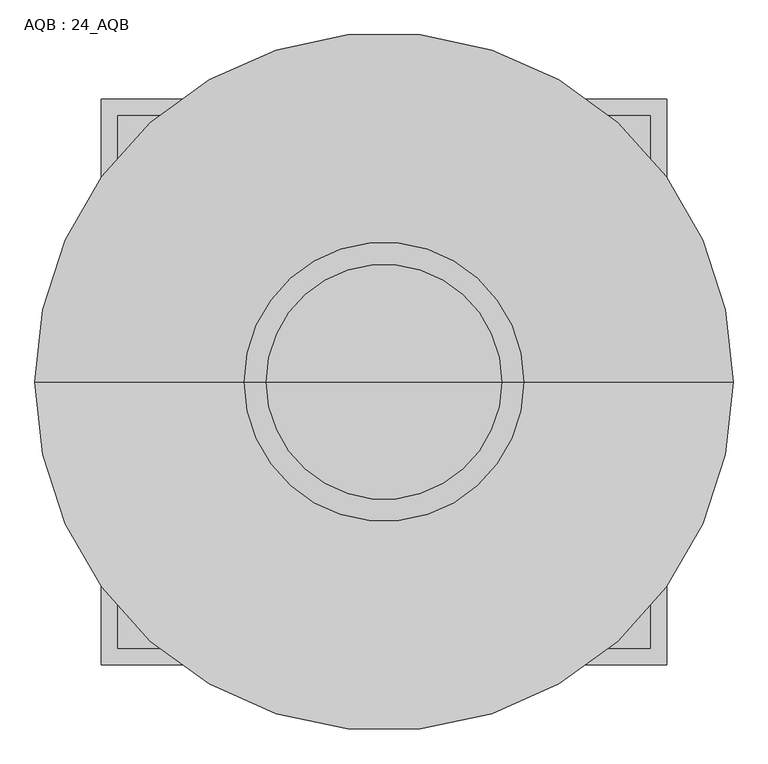
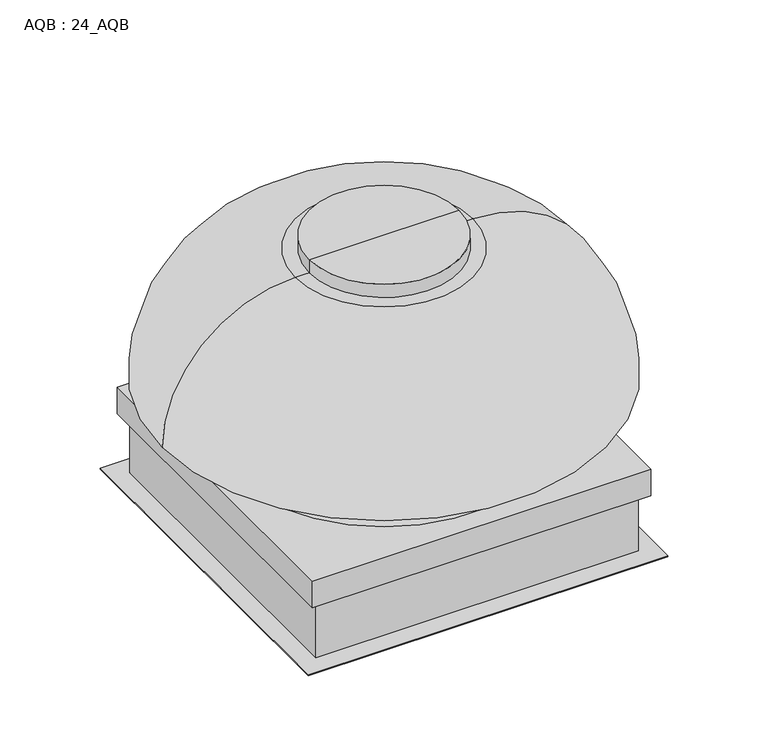
"""IFC4 building model written with IfcOpenShell, lengths in millimetres: proxy geometry, AQB : 24_AQB."""

from ifc_helpers import new_model, si_unit, point, frame, origin, place, context, project, spatial, polyline, circle_curve, ellipse_curve, trimmed, outline, extrude, faceted_brep, source, transform, mapped, element, save
from ifc_brep_helpers import plane_surface, cylinder_surface, revolved_surface, advanced_brep


def aqb_24_aqb_14a4d41b(model_context):
    return source(origin(), model_context, "Body", "SolidModel", [
        extrude(outline(polyline([(499.247472, -488.95), (-478.652528, -488.95), (-478.652528, 488.95), (499.247472, 488.95), (499.247472, -488.95)]), holes=[polyline([(-427.852528, 438.15), (-427.852528, -438.15), (448.447472, -438.15), (448.447472, 438.15), (-427.852528, 438.15)])]), frame((0.0, 0.0, -168.275), z_axis=(0.0, 0.0, 1.0), x_axis=(1.0, 0.0, 0.0)), (0.0, 0.0, 1.0), 3.175),
        extrude(outline(polyline([(-427.852528, 438.15), (448.447472, 438.15), (448.447472, -438.15), (-427.852528, -438.15), (-427.852528, 438.15)]), holes=[polyline([(410.347472, -400.05), (410.347472, 400.05), (-389.752528, 400.05), (-389.752528, -400.05), (410.347472, -400.05)])]), frame((0.0, 0.0, -168.275), z_axis=(0.0, 0.0, 1.0), x_axis=(1.0, 0.0, 0.0)), (0.0, 0.0, 1.0), 241.3),
        advanced_brep(
        [(10.297472, 0.0, 593.725), (-192.902528, 0.0, 593.725), (213.497472, 0.0, 593.725), (213.497472, 0.0, 631.825), (-192.902528, 0.0, 631.825), (10.297472, 0.0, 631.825)],
        [
            (0, 1),
            (1, 2, circle_curve(frame((10.297472, 0.0, 593.725), z_axis=(0.0, 0.0, -1.0), x_axis=(-1.0, 0.0, 0.0)), 203.2)),
            (2, 0),
            (2, 1, circle_curve(frame((10.297472, 0.0, 593.725), z_axis=(0.0, 0.0, -1.0), x_axis=(-1.0, 0.0, 0.0)), 203.2)),
            (3, 4, circle_curve(frame((10.297472, 0.0, 631.825), z_axis=(0.0, 0.0, 1.0), x_axis=(-1.0, 0.0, 0.0)), 203.2)),
            (4, 5),
            (5, 3),
            (4, 3, circle_curve(frame((10.297472, 0.0, 631.825), z_axis=(0.0, 0.0, 1.0), x_axis=(-1.0, 0.0, 0.0)), 203.2)),
            (1, 4),
            (3, 2),
        ],
        [
            plane_surface(frame((10.297472, 0.0, 593.725), z_axis=(0.0, 0.0, -1.0), x_axis=(-1.0, 0.0, 0.0))),
            plane_surface(frame((10.297472, 0.0, 631.825), z_axis=(0.0, 0.0, 1.0), x_axis=(-1.0, 0.0, 0.0))),
            cylinder_surface(frame((10.297472, 0.0, 593.725), z_axis=(0.0, 0.0, -1.0), x_axis=(-1.0, 0.0, 0.0)), 203.2),
        ],
        [
            (0, [[1, 2, 3]]),
            (0, [[-3, 4, -1]]),
            (1, [[5, 6, 7]]),
            (1, [[8, -7, -6]]),
            (2, [[-2, 9, -5, 10]]),
            (2, [[-4, -10, -8, -9]]),
        ],
    ),
        advanced_brep(
        [(10.297472, 0.0, 231.775), (-592.952528, 0.0, 231.775), (613.547472, 0.0, 231.775), (251.597472, 0.0, 593.725), (-231.002528, 0.0, 593.725), (10.297472, 0.0, 593.725)],
        [
            (0, 1),
            (1, 2, circle_curve(frame((10.297472, 0.0, 231.775), z_axis=(0.0, 0.0, -1.0), x_axis=(-1.0, 0.0, 0.0)), 603.25)),
            (2, 0),
            (2, 1, circle_curve(frame((10.297472, 0.0, 231.775), z_axis=(0.0, 0.0, -1.0), x_axis=(-1.0, 0.0, 0.0)), 603.25)),
            (3, 4, circle_curve(frame((10.297472, 0.0, 593.725), z_axis=(0.0, 0.0, 1.0), x_axis=(-1.0, 0.0, 0.0)), 241.3)),
            (4, 5),
            (5, 3),
            (4, 3, circle_curve(frame((10.297472, 0.0, 593.725), z_axis=(0.0, 0.0, 1.0), x_axis=(-1.0, 0.0, 0.0)), 241.3)),
            (1, 4, circle_curve(frame((-231.002528, 0.0, 231.775), z_axis=(0.0, 1.0, 0.0), x_axis=(1.0, 0.0, 0.0)), 361.95)),
            (3, 2, circle_curve(frame((251.597472, 0.0, 231.775), z_axis=(0.0, 1.0, 0.0), x_axis=(-1.0, 0.0, 0.0)), 361.95)),
        ],
        [
            plane_surface(frame((10.297472, 0.0, 231.775), z_axis=(0.0, 0.0, -1.0), x_axis=(-1.0, 0.0, 0.0))),
            plane_surface(frame((10.297472, 0.0, 593.725), z_axis=(0.0, 0.0, 1.0), x_axis=(-1.0, 0.0, 0.0))),
            revolved_surface(trimmed(ellipse_curve(frame((-231.002528, 0.0, 231.775), z_axis=(0.0, -1.0, 0.0), x_axis=(1.0, 0.0, 0.0)), 361.95, 361.95), [point((-231.002528, 0.0, 593.725))], [point((-592.952528, 0.0, 231.775))], True, "CARTESIAN"), (10.297472, 0.0, 593.725), (0.0, 0.0, -1.0)),
        ],
        [
            (0, [[1, 2, 3]]),
            (0, [[-3, 4, -1]]),
            (1, [[5, 6, 7]]),
            (1, [[8, -7, -6]]),
            (2, [[-2, 9, -5, 10]]),
            (2, [[-4, -10, -8, -9]]),
        ],
    ),
        advanced_brep(
        [(416.697472, 0.0, 231.775), (-396.102528, 0.0, 231.775), (10.297472, 0.0, 231.775), (416.697472, 0.0, 76.2), (-396.102528, 0.0, 76.2), (10.297472, 0.0, 76.2)],
        [
            (0, 1, circle_curve(frame((10.297472, 0.0, 231.775), z_axis=(0.0, 0.0, 1.0), x_axis=(-1.0, 0.0, 0.0)), 406.4)),
            (1, 2),
            (2, 0),
            (1, 0, circle_curve(frame((10.297472, 0.0, 231.775), z_axis=(0.0, 0.0, 1.0), x_axis=(-1.0, 0.0, 0.0)), 406.4)),
            (3, 4, circle_curve(frame((10.297472, 0.0, 76.2), z_axis=(0.0, 0.0, 1.0), x_axis=(-1.0, 0.0, 0.0)), 406.4)),
            (4, 1, circle_curve(frame((-396.102528, 0.0, 153.9875), z_axis=(0.0, -1.0, 0.0), x_axis=(1.0, 0.0, 0.0)), 77.7875)),
            (0, 3, circle_curve(frame((416.697472, 0.0, 153.9875), z_axis=(0.0, -1.0, 0.0), x_axis=(-1.0, 0.0, 0.0)), 77.7875)),
            (4, 3, circle_curve(frame((10.297472, 0.0, 76.2), z_axis=(0.0, 0.0, 1.0), x_axis=(-1.0, 0.0, 0.0)), 406.4)),
            (5, 4),
            (3, 5),
        ],
        [
            plane_surface(frame((10.297472, 0.0, 231.775), z_axis=(0.0, 0.0, 1.0), x_axis=(-1.0, 0.0, 0.0))),
            revolved_surface(trimmed(ellipse_curve(frame((-396.102528, 0.0, 153.9875), z_axis=(0.0, 1.0, 0.0), x_axis=(1.0, 0.0, 0.0)), 77.7875, 77.7875), [point((-396.102528, 0.0, 231.775))], [point((-396.102528, 0.0, 76.2))], True, "CARTESIAN"), (10.297472, 0.0, 76.2), (0.0, 0.0, -1.0)),
            plane_surface(frame((10.297472, 0.0, 76.2), z_axis=(0.0, 0.0, -1.0), x_axis=(-1.0, 0.0, 0.0))),
        ],
        [
            (0, [[1, 2, 3]]),
            (0, [[4, -3, -2]]),
            (1, [[5, 6, -1, 7]]),
            (1, [[8, -7, -4, -6]]),
            (2, [[9, -5, 10]]),
            (2, [[-10, -8, -9]]),
        ],
    ),
        faceted_brep([(470.672472, 460.375, 76.2), (-450.077528, 460.375, 76.2), (-450.077528, -460.375, 76.2), (470.672472, -460.375, 76.2), (470.672472, 460.375, 0.0), (470.672472, -460.375, 0.0), (-450.077528, -460.375, 0.0), (-450.077528, 460.375, 0.0), (467.497472, 457.2, 0.0), (-446.902528, 457.2, 0.0), (-446.902528, -457.2, 0.0), (467.497472, -457.2, 0.0), (467.497472, 457.2, 73.025), (467.497472, -457.2, 73.025), (-446.902528, -457.2, 73.025), (-446.902528, 457.2, 73.025)], [[[0, 1, 2, 3]], [[4, 5, 6, 7], [8, 9, 10, 11]], [[1, 0, 4, 7]], [[2, 1, 7, 6]], [[3, 2, 6, 5]], [[0, 3, 5, 4]], [[12, 13, 14, 15]], [[12, 15, 9, 8]], [[15, 14, 10, 9]], [[14, 13, 11, 10]], [[13, 12, 8, 11]]]),
    ])


if __name__ == "__main__":
    model = new_model("IFC4")
    model_context = context("Model", 3, world=origin())
    ifc_project = project(units=[si_unit("LENGTHUNIT", "METRE", prefix="MILLI")], contexts=[model_context])
    site = spatial("IfcSite", under=ifc_project)
    building = spatial("IfcBuilding", under=site)
    placement = place(None, origin())
    aqb_24_aqb_shape = aqb_24_aqb_14a4d41b(model_context)
    element("IfcBuildingElementProxy", 1, Name="AQB : 24_AQB", ObjectType="AQB : 24_AQB", at=placement, inside=building, context=model_context, shape_type="MappedRepresentation", body=[
        mapped(aqb_24_aqb_shape, transform((0.0, 0.0, 0.0), x_axis=(1.0, 0.0, 0.0), y_axis=(0.0, 1.0, 0.0), z_axis=(0.0, 0.0, 1.0))),
    ])
    save(model, "model.ifc")

# Revit data of these elements
# Type "AQB : 24_AQB"
#   bim-seek-source_url = ""
#   Youtube clip = ""
#   Unit Weight [instance default] = ""
#   Uniclass 2015 Name = ""
#   Uniclass 2015 Code = ""
#   Uniclass 2.0 Description = "Air Vents"
#   Uniclass 2.0 Code = "PR-94-93-xx"
#   Uniclass 1.4 Description = ""
#   Uniclass 1.4 Code = ""
#   UNSPSC Code = "40101502"
#   Technical description = ""
#   Sones [instance default] = ""
#   Region South America = "None"
#   Region Oceania = "None"
#   Region North America = "US"
#   Region Middle East = "None"
#   Region Europe = "None"
#   Region Asia = "None"
#   Region Antarctica = "None"
#   Region Africa = "None"
#   QR code = ""
#   Product group = "Exhaust"
#   Product family = "Air Condition Equipment"
#   Product data url = ""
#   Product certification = ""
#   Product SKU = "roofexhaustfan"
#   Product Guid = ""
#   OmniClass Description = ""
#   OmniClass Code = ""
#   NBS Reference Description = "Air Vents"
#   NBS Reference Code = "94-93-xx"
#   Motor RPM [instance default] = ""
#   Motor Enclosure [instance default] = ""
#   Material secondary = ""
#   Material main = "Aluminium"
#   Manufacturer name = "Loren Cook Company"
#   Manufacturer country = "United States"
#   LwA [instance default] = ""
#   Installation instructions = ""
#   IFC Classification = "Roof"
#   Fan RPM [instance default] = ""
#   EAN code = ""
#   Design country = "United States"
#   Date of publishing = "4/1/2014"
#   COBIe Type Category = ""
#   BIMobject category = "Mechanical Ventilation"
#   Brake Hp [instance default] = ""
#   Type Comments = "Downblast Propeller Exhaust Ventilator Roof Mounted/Belt Drive"
#   Motor Hp [instance default] = "0"
#   Model = "AQB"
#   Weight Net (Kg) = 0
#   T_SQ/2+.125" = 0.460375 m
#   RO/2 = 0.40005 m
#   Nominal width = 0
#   Nominal height = 0
#   RO = 0.8001 m
#   T_SQ/2 = 0.4572 m
#   T_SQ = 0.9144 m
#   D/2-(A-B) = 0.2032 m
#   C_ = 1.2065 m
#   C_/2 = 0.60325 m
#   CURB_HEIGHT [instance default] = 0.2413 m
#   BASE-.125 = 0.073025 m
#   BASE = 0.0762 m
#   B/2 = 0.115888 m
#   B-C/2 = 0.077787 m
#   B-C = 0.155575 m
#   B = 0.231775 m
#   A/2 = 0.315912 m
#   A-B = 0.40005 m
#   A-1.5" = 0.593725 m
#   A = 0.631825 m
#   4" = 0.1016 m
#   2' = 0.6096 m
#   2" = 0.0508 m
#   1" = 0.0254 m
#   0 = 0.0000 m
#   Voltage [instance default] = 0 V
#   Static Pressure [instance default] = 0.0 Pa
#   Power [instance default] = 0 W
#   Motor FLA [instance default] = 0 A
#   CFM [instance default] = 0.0 L/s
#   1.5 = 0.0381 m
#   .125 = 0.003175 m
#   -(C/2) = -0.0381 m
#   -(A/2) = -0.315912 m
#   (T_SQ/2)-2" = 0.4064 m
#   bim-seek-BOPCEditionNumber = 1
#   Edition number = 1
#   CURB [instance default] = yes
#   Phase [instance default] = 0
#   Number of Poles [instance default] = 1
#   Default Elevation = 0
#   URL = ""
#   Manufacturer = ""
